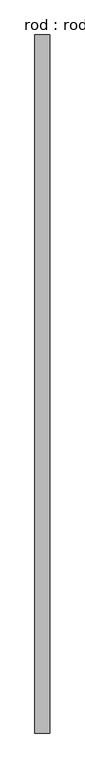
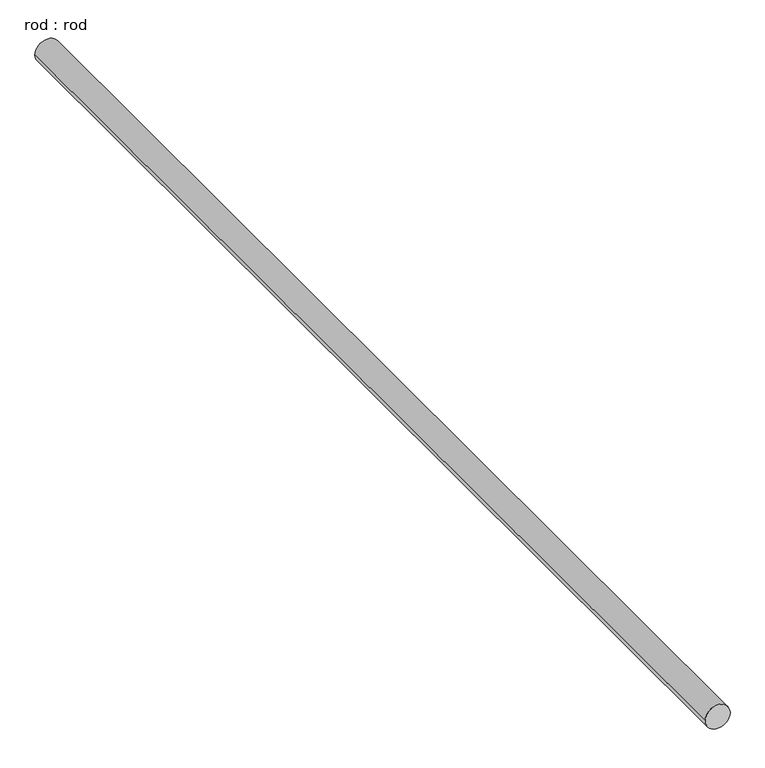
"""IFC4 building model written with IfcOpenShell, lengths in millimetres: proxy geometry, rod : rod."""

import ifcopenshell
import ifcopenshell.guid

model = None  # the IFC model being written
_history = None  # IfcOwnerHistory: only IFC2X3 demands one
_inside = {}  # id of a spatial element -> (the spatial element, [elements in it])
_under = {}  # id of a project, library or spatial element -> (it, [spatial elements below it])
_declared = {}  # id of a project -> (the project, [libraries it declares])
_typed = {}  # id of a type object -> (the type object, [elements of that type])
_made_of = {}  # id of a material, layer set ... -> (it, [elements and type objects made of it])


def new_model(schema):
    """Start an empty IFC model of exactly this schema.

    Asked for "IFC4X3", IfcOpenShell would pick the latest addendum, in which some entities
    have other attributes; the version numbers below select the first issue.
    IFC2X3 requires an IfcOwnerHistory on every rooted entity: one is made here for all.
    """
    global model, _history
    if schema == "IFC4X3":
        model = ifcopenshell.file(schema_version=(4, 3, 0, 0))
    else:
        model = ifcopenshell.file(schema=schema)
    _inside.clear()
    _under.clear()
    _declared.clear()
    _typed.clear()
    _made_of.clear()
    _history = None
    if model.schema == "IFC2X3":
        org = make("IfcOrganization", Name="unknown")
        user = make(
            "IfcPersonAndOrganization",
            ThePerson=make("IfcPerson", FamilyName="unknown"),
            TheOrganization=org,
        )
        app = make(
            "IfcApplication",
            ApplicationDeveloper=org,
            Version="unknown",
            ApplicationFullName="unknown",
            ApplicationIdentifier="unknown",
        )
        _history = make(
            "IfcOwnerHistory",
            OwningUser=user,
            OwningApplication=app,
            ChangeAction="ADDED",
            CreationDate=0,
        )
    return model


def make(cls, **values):
    """One entity of the class cls with the attributes given. An attribute that is None is left unset."""
    return model.create_entity(
        cls, **{name: value for name, value in values.items() if value is not None}
    )


def rooted(cls, **values):
    """An entity with a GlobalId (a new one), such as an element, a storey or a relation."""
    return make(cls, GlobalId=ifcopenshell.guid.new(), OwnerHistory=_history, **values)


def si_unit(unit_type, name, prefix=None):
    """IfcSIUnit, for example si_unit("LENGTHUNIT", "METRE", prefix="MILLI")."""
    return make("IfcSIUnit", UnitType=unit_type, Prefix=prefix, Name=name)


def assignment(units):
    """IfcUnitAssignment: the units of a project."""
    return None if units is None else make("IfcUnitAssignment", Units=units)


def point(xyz):
    """IfcCartesianPoint."""
    return None if xyz is None else make("IfcCartesianPoint", Coordinates=xyz)


def direction(xyz):
    """IfcDirection."""
    return None if xyz is None else make("IfcDirection", DirectionRatios=xyz)


def frame(location, z_axis=None, x_axis=None):
    """IfcAxis2Placement3D, a coordinate frame: its origin and axes. An axis left out is left unset."""
    return make(
        "IfcAxis2Placement3D",
        Location=point(location),
        Axis=direction(z_axis),
        RefDirection=direction(x_axis),
    )


def frame_2d(location, x_axis=None):
    """IfcAxis2Placement2D, a coordinate frame in the plane: its origin and x axis."""
    return make(
        "IfcAxis2Placement2D", Location=point(location), RefDirection=direction(x_axis)
    )


def origin():
    """The frame at (0, 0, 0) with its axes left unset."""
    return frame((0.0, 0.0, 0.0))


def place(relative_to, where):
    """IfcLocalPlacement: puts the frame where relative to a parent placement (None: the world)."""
    return make(
        "IfcLocalPlacement", PlacementRelTo=relative_to, RelativePlacement=where
    )


def context(
    kind, dimensions, precision=None, world=None, true_north=None, identifier=None
):
    """IfcGeometricRepresentationContext, for example the 3D "Model" context."""
    return make(
        "IfcGeometricRepresentationContext",
        ContextIdentifier=identifier,
        ContextType=kind,
        CoordinateSpaceDimension=dimensions,
        Precision=precision,
        WorldCoordinateSystem=world,
        TrueNorth=true_north,
    )


def project(units=None, contexts=None):
    """IfcProject with its units and contexts."""
    return rooted(
        "IfcProject",
        Name="project",
        RepresentationContexts=contexts,
        UnitsInContext=assignment(units),
    )


def spatial(cls, under=None, at=None, **own):
    """A site, building, storey or space (cls), placed at a placement, below another one or the project."""
    s = rooted(cls, ObjectPlacement=at, **own)
    if under is not None:
        _under.setdefault(under.id(), (under, []))[1].append(s)
    return s


def circle_curve(where, radius):
    """IfcCircle in the frame where."""
    return make("IfcCircle", Position=where, Radius=radius)


def trimmed(basis, trim1, trim2, sense, master):
    """IfcTrimmedCurve: the piece of a basis curve between two trims."""
    return make(
        "IfcTrimmedCurve",
        BasisCurve=basis,
        Trim1=trim1,
        Trim2=trim2,
        SenseAgreement=sense,
        MasterRepresentation=master,
    )


def segment(curve, same_sense, transition):
    """IfcCompositeCurveSegment."""
    return make(
        "IfcCompositeCurveSegment",
        Transition=transition,
        SameSense=same_sense,
        ParentCurve=curve,
    )


def composite_curve(segments, self_intersect=None):
    """IfcCompositeCurve: segments joined end to end."""
    return make("IfcCompositeCurve", Segments=segments, SelfIntersect=self_intersect)


def outline(outer, holes=None, kind="AREA"):
    """IfcArbitraryClosedProfileDef: a profile drawn as a closed curve; with holes, ...WithVoids."""
    if holes is None:
        return make("IfcArbitraryClosedProfileDef", ProfileType=kind, OuterCurve=outer)
    return make(
        "IfcArbitraryProfileDefWithVoids",
        ProfileType=kind,
        OuterCurve=outer,
        InnerCurves=holes,
    )


def extrude(swept, where, along, depth):
    """IfcExtrudedAreaSolid: the profile swept, set in the frame where, extruded along a direction by depth."""
    return make(
        "IfcExtrudedAreaSolid",
        SweptArea=swept,
        Position=where,
        ExtrudedDirection=direction(along),
        Depth=depth,
    )


def shape(context_of_items, identifier, shape_type, items):
    """IfcShapeRepresentation: the items that make up one representation, for example the "Body"."""
    return make(
        "IfcShapeRepresentation",
        ContextOfItems=context_of_items,
        RepresentationIdentifier=identifier,
        RepresentationType=shape_type,
        Items=items,
    )


def source(mapping_origin, context_of_items, identifier, shape_type, items):
    """IfcRepresentationMap: a shape defined once, which mapped items show again and again."""
    return make(
        "IfcRepresentationMap",
        MappingOrigin=mapping_origin,
        MappedRepresentation=shape(context_of_items, identifier, shape_type, items),
    )


def transform(
    local_origin,
    x_axis=None,
    y_axis=None,
    z_axis=None,
    scale=None,
    scale2=None,
    scale3=None,
    uniform=True,
):
    """IfcCartesianTransformationOperator3D, or its non-uniform kind. x_axis, y_axis, z_axis: its Axis1, 2, 3."""
    if uniform:
        return make(
            "IfcCartesianTransformationOperator3D",
            Axis1=direction(x_axis),
            Axis2=direction(y_axis),
            LocalOrigin=point(local_origin),
            Scale=scale,
            Axis3=direction(z_axis),
        )
    return make(
        "IfcCartesianTransformationOperator3DnonUniform",
        Axis1=direction(x_axis),
        Axis2=direction(y_axis),
        LocalOrigin=point(local_origin),
        Scale=scale,
        Axis3=direction(z_axis),
        Scale2=scale2,
        Scale3=scale3,
    )


def mapped(mapping_source, mapping_target):
    """IfcMappedItem: shows the shape of a source again, moved by a transform."""
    return make(
        "IfcMappedItem", MappingSource=mapping_source, MappingTarget=mapping_target
    )


def made_of(thing, what):
    """Note that an element or type object is made of a material, layer set ...; save() writes the relation."""
    if what is not None:
        _made_of.setdefault(what.id(), (what, []))[1].append(thing)
    return thing


def element(
    cls,
    number,
    at=None,
    inside=None,
    cuts=None,
    type_object=None,
    material=None,
    context=None,
    identifier="Body",
    shape_type=None,
    held_by="IfcProductDefinitionShape",
    body=None,
    shapes=None,
    **own,
):
    """One element of the class cls, such as IfcWall. Its Tag is "e" and its number.

    at: its placement. inside: the storey or other place that contains it. cuts: it is an
    opening in that element (IfcRelVoidsElement). A single representation is given by context,
    identifier, shape_type and body (its items); several are given by shapes. held_by: the class
    of the entity that holds the representations. save() writes the other relations.
    """
    e = rooted(cls, Tag="e%d" % number, ObjectPlacement=at, **own)
    if body is not None:
        shapes = [shape(context, identifier, shape_type, body)]
    if shapes is not None:
        e.Representation = make(held_by, Representations=shapes)
    if inside is not None:
        _inside.setdefault(inside.id(), (inside, []))[1].append(e)
    if cuts is not None:
        rooted(
            "IfcRelVoidsElement", RelatingBuildingElement=cuts, RelatedOpeningElement=e
        )
    if type_object is not None:
        _typed.setdefault(type_object.id(), (type_object, []))[1].append(e)
    return made_of(e, material)


def aggregate(whole, parts):
    """IfcRelAggregates: a whole, such as a stair, and the parts it consists of."""
    return rooted("IfcRelAggregates", RelatingObject=whole, RelatedObjects=parts)


def save(model, path):
    """Write the relations noted so far, then the file.

    IfcRelAggregates (storeys below a building ...), IfcRelContainedInSpatialStructure (elements
    in a storey), IfcRelDefinesByType, IfcRelAssociatesMaterial and IfcRelDeclares: one each for
    every whole, place, type object, material and project.
    """
    for whole, parts in _under.values():
        aggregate(whole, parts)
    for where, things in _inside.values():
        rooted(
            "IfcRelContainedInSpatialStructure",
            RelatedElements=things,
            RelatingStructure=where,
        )
    for kind, things in _typed.values():
        rooted("IfcRelDefinesByType", RelatedObjects=things, RelatingType=kind)
    for what, things in _made_of.values():
        rooted("IfcRelAssociatesMaterial", RelatedObjects=things, RelatingMaterial=what)
    for by, libraries in _declared.values():
        rooted("IfcRelDeclares", RelatingContext=by, RelatedDefinitions=libraries)
    model.write(path)


def rod_rod_ca46379e(model_context):
    return source(origin(), model_context, "Body", "SweptSolid", [
        extrude(outline(composite_curve([segment(trimmed(circle_curve(frame_2d((0.0108462, 0.0)), 200.0), [point((0.0108462, 200.0))], [point((0.0108462, -200.0))], False, "CARTESIAN"), True, "CONTINUOUS"), segment(trimmed(circle_curve(frame_2d((0.0108462, 0.0)), 200.0), [point((0.0108462, -200.0))], [point((0.0108462, 200.0))], False, "CARTESIAN"), True, "CONTINUOUS")], self_intersect=False)), frame((0.0, -5213.194263, 0.0), z_axis=(0.0, 1.0, 0.0), x_axis=(0.0, 0.0, 1.0)), (0.0, 0.0, 1.0), 18611.8457566),
    ])


if __name__ == "__main__":
    model = new_model("IFC4")
    model_context = context("Model", 3, world=origin())
    ifc_project = project(units=[si_unit("LENGTHUNIT", "METRE", prefix="MILLI")], contexts=[model_context])
    site = spatial("IfcSite", under=ifc_project)
    building = spatial("IfcBuilding", under=site)
    placement = place(None, origin())
    rod_rod_shape = rod_rod_ca46379e(model_context)
    element("IfcBuildingElementProxy", 1, Name="rod : rod", ObjectType="rod : rod", at=placement, inside=building, context=model_context, shape_type="MappedRepresentation", body=[
        mapped(rod_rod_shape, transform((0.0, 0.0, 0.0), x_axis=(1.0, 0.0, 0.0), y_axis=(0.0, 1.0, 0.0), z_axis=(0.0, 0.0, 1.0))),
    ])
    save(model, "model.ifc")

# Revit data of these elements
# Type "rod : rod"
#   Default Elevation = 0
